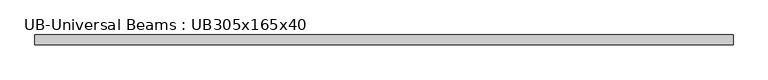
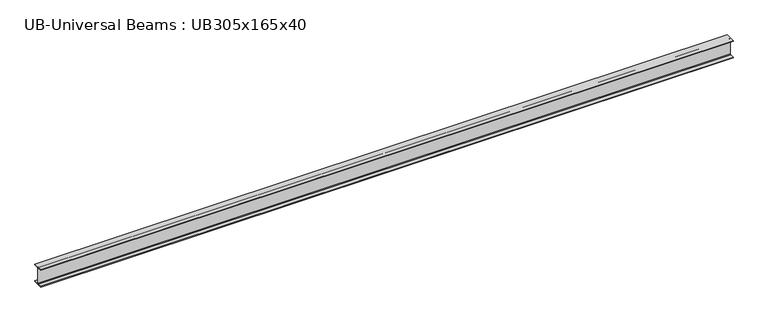
"""IFC4 building model written with IfcOpenShell, lengths in millimetres: member geometry, UB-Universal Beams : UB305x165x40."""

from ifc_helpers import new_model, si_unit, point, frame, frame_2d, origin, place, context, project, spatial, polyline, circle_curve, trimmed, segment, composite_curve, outline, extrude, source, transform, mapped, element, save


def ub_universal_beams_ub305x165x40_c2663d37(model_context):
    return source(origin(), model_context, "Body", "SweptSolid", [
        extrude(outline(composite_curve([segment(polyline([(82.5, -141.5), (82.5, -151.7), (-82.5, -151.7), (-82.5, -141.5), (-11.9, -141.5)]), True, "CONTINUOUS"), segment(trimmed(circle_curve(frame_2d((-11.9, -132.6)), 8.9), [point((-11.9, -141.5))], [point((-3.0, -132.6))], True, "CARTESIAN"), True, "CONTINUOUS"), segment(polyline([(-3.0, -132.6), (-3.0, 132.6)]), True, "CONTINUOUS"), segment(trimmed(circle_curve(frame_2d((-11.9, 132.6)), 8.9), [point((-3.0, 132.6))], [point((-11.9, 141.5))], True, "CARTESIAN"), True, "CONTINUOUS"), segment(polyline([(-11.9, 141.5), (-82.5, 141.5), (-82.5, 151.7), (82.5, 151.7), (82.5, 141.5), (11.9, 141.5)]), True, "CONTINUOUS"), segment(trimmed(circle_curve(frame_2d((11.9, 132.6)), 8.9), [point((11.9, 141.5))], [point((3.0, 132.6))], True, "CARTESIAN"), True, "CONTINUOUS"), segment(polyline([(3.0, 132.6), (3.0, -132.6)]), True, "CONTINUOUS"), segment(trimmed(circle_curve(frame_2d((11.9, -132.6)), 8.9), [point((3.0, -132.6))], [point((11.9, -141.5))], True, "CARTESIAN"), True, "CONTINUOUS"), segment(polyline([(11.9, -141.5), (82.5, -141.5)]), True, "CONTINUOUS")], self_intersect=False)), frame((-5634.75, 0.0, 0.0), z_axis=(1.0, 0.0, 0.0), x_axis=(0.0, 1.0, 0.0)), (0.0, 0.0, 1.0), 11590.6),
    ])


if __name__ == "__main__":
    model = new_model("IFC4")
    model_context = context("Model", 3, world=origin())
    ifc_project = project(units=[si_unit("LENGTHUNIT", "METRE", prefix="MILLI")], contexts=[model_context])
    site = spatial("IfcSite", under=ifc_project)
    building = spatial("IfcBuilding", under=site)
    placement = place(None, origin())
    ub_universal_beams_ub305x165x40_shape = ub_universal_beams_ub305x165x40_c2663d37(model_context)
    element("IfcMember", 1, ObjectType="UB-Universal Beams : UB305x165x40", at=placement, inside=building, context=model_context, shape_type="MappedRepresentation", body=[
        mapped(ub_universal_beams_ub305x165x40_shape, transform((0.0, 0.0, 0.0), x_axis=(1.0, 0.0, 0.0), y_axis=(0.0, 1.0, 0.0), z_axis=(0.0, 0.0, 1.0))),
    ])
    save(model, "model.ifc")

# Revit data of these elements
# Type "UB-Universal Beams : UB305x165x40"
#   Section Name Key = "UB305X165X40"
#   Width = 16.5 cm
#   Web Thickness = 0.6 cm
#   Web Fillet = 0.89 cm
#   Warping Constant = 164000.0 cm⁶
#   Torsional Moment of Inertia = 14.70 cm⁴
#   Section Area = 51.3 cm²
#   Plastic Modulus weak axis = 142.0 cm³
#   Plastic Modulus strong axis = 623.0 cm³
#   Nominal Weight = 40.2999 kgf/m
#   Moment of Inertia weak axis = 764.00 cm⁴
#   Moment of Inertia strong axis = 8503.00 cm⁴
#   Height = 30.34 cm
#   Flange Thickness = 1.02 cm
#   Elastic Modulus weak axis = 92.6 cm³
#   Elastic Modulus strong axis = 560.0 cm³
#   Centroid Vertical = 15.17 cm
#   Centroid Horizontal = 8.25 cm
#   Bolt Spacing = 9.0 cm
#   Length [instance default] = 1500 mm
#   Structural Material [instance default] = Metal - Steel 43-275
#   Type Comments = ""
#   Assembly Code = ""
# Element 1 (IfcMember, "UB-Universal Beams : UB305x165x40")
#   Materials on its faces: "Metal - Steel 43-275"
# Materials
#   "Metal - Steel 43-275": class "Metal", colour RGB 247 247 247, transparency 0, Cost = 0
